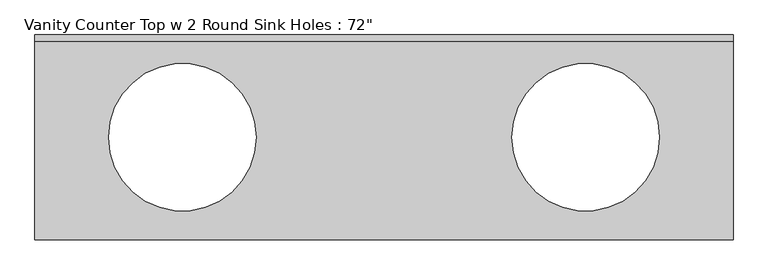
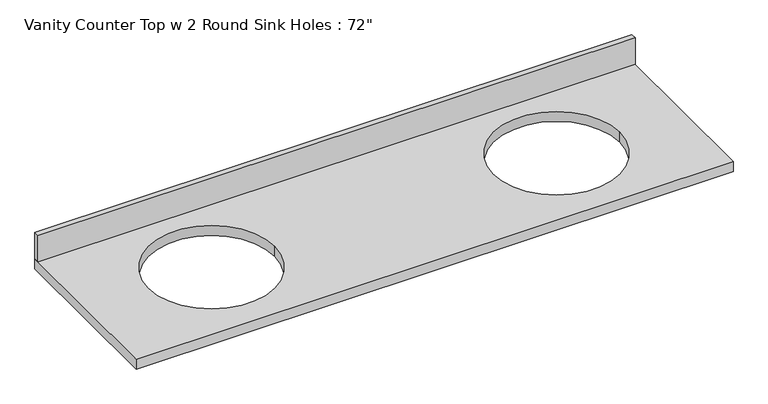
"""IFC4 building model written with IfcOpenShell, lengths in millimetres: furniture geometry."""

import ifcopenshell
import ifcopenshell.guid

model = None  # the IFC model being written
_history = None  # IfcOwnerHistory: only IFC2X3 demands one
_inside = {}  # id of a spatial element -> (the spatial element, [elements in it])
_under = {}  # id of a project, library or spatial element -> (it, [spatial elements below it])
_declared = {}  # id of a project -> (the project, [libraries it declares])
_typed = {}  # id of a type object -> (the type object, [elements of that type])
_made_of = {}  # id of a material, layer set ... -> (it, [elements and type objects made of it])


def new_model(schema):
    """Start an empty IFC model of exactly this schema.

    Asked for "IFC4X3", IfcOpenShell would pick the latest addendum, in which some entities
    have other attributes; the version numbers below select the first issue.
    IFC2X3 requires an IfcOwnerHistory on every rooted entity: one is made here for all.
    """
    global model, _history
    if schema == "IFC4X3":
        model = ifcopenshell.file(schema_version=(4, 3, 0, 0))
    else:
        model = ifcopenshell.file(schema=schema)
    _inside.clear()
    _under.clear()
    _declared.clear()
    _typed.clear()
    _made_of.clear()
    _history = None
    if model.schema == "IFC2X3":
        org = make("IfcOrganization", Name="unknown")
        user = make(
            "IfcPersonAndOrganization",
            ThePerson=make("IfcPerson", FamilyName="unknown"),
            TheOrganization=org,
        )
        app = make(
            "IfcApplication",
            ApplicationDeveloper=org,
            Version="unknown",
            ApplicationFullName="unknown",
            ApplicationIdentifier="unknown",
        )
        _history = make(
            "IfcOwnerHistory",
            OwningUser=user,
            OwningApplication=app,
            ChangeAction="ADDED",
            CreationDate=0,
        )
    return model


def make(cls, **values):
    """One entity of the class cls with the attributes given. An attribute that is None is left unset."""
    return model.create_entity(
        cls, **{name: value for name, value in values.items() if value is not None}
    )


def rooted(cls, **values):
    """An entity with a GlobalId (a new one), such as an element, a storey or a relation."""
    return make(cls, GlobalId=ifcopenshell.guid.new(), OwnerHistory=_history, **values)


def si_unit(unit_type, name, prefix=None):
    """IfcSIUnit, for example si_unit("LENGTHUNIT", "METRE", prefix="MILLI")."""
    return make("IfcSIUnit", UnitType=unit_type, Prefix=prefix, Name=name)


def assignment(units):
    """IfcUnitAssignment: the units of a project."""
    return None if units is None else make("IfcUnitAssignment", Units=units)


def point(xyz):
    """IfcCartesianPoint."""
    return None if xyz is None else make("IfcCartesianPoint", Coordinates=xyz)


def direction(xyz):
    """IfcDirection."""
    return None if xyz is None else make("IfcDirection", DirectionRatios=xyz)


def frame(location, z_axis=None, x_axis=None):
    """IfcAxis2Placement3D, a coordinate frame: its origin and axes. An axis left out is left unset."""
    return make(
        "IfcAxis2Placement3D",
        Location=point(location),
        Axis=direction(z_axis),
        RefDirection=direction(x_axis),
    )


def frame_2d(location, x_axis=None):
    """IfcAxis2Placement2D, a coordinate frame in the plane: its origin and x axis."""
    return make(
        "IfcAxis2Placement2D", Location=point(location), RefDirection=direction(x_axis)
    )


def origin():
    """The frame at (0, 0, 0) with its axes left unset."""
    return frame((0.0, 0.0, 0.0))


def place(relative_to, where):
    """IfcLocalPlacement: puts the frame where relative to a parent placement (None: the world)."""
    return make(
        "IfcLocalPlacement", PlacementRelTo=relative_to, RelativePlacement=where
    )


def context(
    kind, dimensions, precision=None, world=None, true_north=None, identifier=None
):
    """IfcGeometricRepresentationContext, for example the 3D "Model" context."""
    return make(
        "IfcGeometricRepresentationContext",
        ContextIdentifier=identifier,
        ContextType=kind,
        CoordinateSpaceDimension=dimensions,
        Precision=precision,
        WorldCoordinateSystem=world,
        TrueNorth=true_north,
    )


def project(units=None, contexts=None):
    """IfcProject with its units and contexts."""
    return rooted(
        "IfcProject",
        Name="project",
        RepresentationContexts=contexts,
        UnitsInContext=assignment(units),
    )


def spatial(cls, under=None, at=None, **own):
    """A site, building, storey or space (cls), placed at a placement, below another one or the project."""
    s = rooted(cls, ObjectPlacement=at, **own)
    if under is not None:
        _under.setdefault(under.id(), (under, []))[1].append(s)
    return s


def polyline(points):
    """IfcPolyline through the points."""
    return make("IfcPolyline", Points=[point(p) for p in points])


def circle_curve(where, radius):
    """IfcCircle in the frame where."""
    return make("IfcCircle", Position=where, Radius=radius)


def trimmed(basis, trim1, trim2, sense, master):
    """IfcTrimmedCurve: the piece of a basis curve between two trims."""
    return make(
        "IfcTrimmedCurve",
        BasisCurve=basis,
        Trim1=trim1,
        Trim2=trim2,
        SenseAgreement=sense,
        MasterRepresentation=master,
    )


def segment(curve, same_sense, transition):
    """IfcCompositeCurveSegment."""
    return make(
        "IfcCompositeCurveSegment",
        Transition=transition,
        SameSense=same_sense,
        ParentCurve=curve,
    )


def composite_curve(segments, self_intersect=None):
    """IfcCompositeCurve: segments joined end to end."""
    return make("IfcCompositeCurve", Segments=segments, SelfIntersect=self_intersect)


def outline(outer, holes=None, kind="AREA"):
    """IfcArbitraryClosedProfileDef: a profile drawn as a closed curve; with holes, ...WithVoids."""
    if holes is None:
        return make("IfcArbitraryClosedProfileDef", ProfileType=kind, OuterCurve=outer)
    return make(
        "IfcArbitraryProfileDefWithVoids",
        ProfileType=kind,
        OuterCurve=outer,
        InnerCurves=holes,
    )


def extrude(swept, where, along, depth):
    """IfcExtrudedAreaSolid: the profile swept, set in the frame where, extruded along a direction by depth."""
    return make(
        "IfcExtrudedAreaSolid",
        SweptArea=swept,
        Position=where,
        ExtrudedDirection=direction(along),
        Depth=depth,
    )


def shape(context_of_items, identifier, shape_type, items):
    """IfcShapeRepresentation: the items that make up one representation, for example the "Body"."""
    return make(
        "IfcShapeRepresentation",
        ContextOfItems=context_of_items,
        RepresentationIdentifier=identifier,
        RepresentationType=shape_type,
        Items=items,
    )


def source(mapping_origin, context_of_items, identifier, shape_type, items):
    """IfcRepresentationMap: a shape defined once, which mapped items show again and again."""
    return make(
        "IfcRepresentationMap",
        MappingOrigin=mapping_origin,
        MappedRepresentation=shape(context_of_items, identifier, shape_type, items),
    )


def transform(
    local_origin,
    x_axis=None,
    y_axis=None,
    z_axis=None,
    scale=None,
    scale2=None,
    scale3=None,
    uniform=True,
):
    """IfcCartesianTransformationOperator3D, or its non-uniform kind. x_axis, y_axis, z_axis: its Axis1, 2, 3."""
    if uniform:
        return make(
            "IfcCartesianTransformationOperator3D",
            Axis1=direction(x_axis),
            Axis2=direction(y_axis),
            LocalOrigin=point(local_origin),
            Scale=scale,
            Axis3=direction(z_axis),
        )
    return make(
        "IfcCartesianTransformationOperator3DnonUniform",
        Axis1=direction(x_axis),
        Axis2=direction(y_axis),
        LocalOrigin=point(local_origin),
        Scale=scale,
        Axis3=direction(z_axis),
        Scale2=scale2,
        Scale3=scale3,
    )


def mapped(mapping_source, mapping_target):
    """IfcMappedItem: shows the shape of a source again, moved by a transform."""
    return make(
        "IfcMappedItem", MappingSource=mapping_source, MappingTarget=mapping_target
    )


def made_of(thing, what):
    """Note that an element or type object is made of a material, layer set ...; save() writes the relation."""
    if what is not None:
        _made_of.setdefault(what.id(), (what, []))[1].append(thing)
    return thing


def element(
    cls,
    number,
    at=None,
    inside=None,
    cuts=None,
    type_object=None,
    material=None,
    context=None,
    identifier="Body",
    shape_type=None,
    held_by="IfcProductDefinitionShape",
    body=None,
    shapes=None,
    **own,
):
    """One element of the class cls, such as IfcWall. Its Tag is "e" and its number.

    at: its placement. inside: the storey or other place that contains it. cuts: it is an
    opening in that element (IfcRelVoidsElement). A single representation is given by context,
    identifier, shape_type and body (its items); several are given by shapes. held_by: the class
    of the entity that holds the representations. save() writes the other relations.
    """
    e = rooted(cls, Tag="e%d" % number, ObjectPlacement=at, **own)
    if body is not None:
        shapes = [shape(context, identifier, shape_type, body)]
    if shapes is not None:
        e.Representation = make(held_by, Representations=shapes)
    if inside is not None:
        _inside.setdefault(inside.id(), (inside, []))[1].append(e)
    if cuts is not None:
        rooted(
            "IfcRelVoidsElement", RelatingBuildingElement=cuts, RelatedOpeningElement=e
        )
    if type_object is not None:
        _typed.setdefault(type_object.id(), (type_object, []))[1].append(e)
    return made_of(e, material)


def aggregate(whole, parts):
    """IfcRelAggregates: a whole, such as a stair, and the parts it consists of."""
    return rooted("IfcRelAggregates", RelatingObject=whole, RelatedObjects=parts)


def save(model, path):
    """Write the relations noted so far, then the file.

    IfcRelAggregates (storeys below a building ...), IfcRelContainedInSpatialStructure (elements
    in a storey), IfcRelDefinesByType, IfcRelAssociatesMaterial and IfcRelDeclares: one each for
    every whole, place, type object, material and project.
    """
    for whole, parts in _under.values():
        aggregate(whole, parts)
    for where, things in _inside.values():
        rooted(
            "IfcRelContainedInSpatialStructure",
            RelatedElements=things,
            RelatingStructure=where,
        )
    for kind, things in _typed.values():
        rooted("IfcRelDefinesByType", RelatedObjects=things, RelatingType=kind)
    for what, things in _made_of.values():
        rooted("IfcRelAssociatesMaterial", RelatedObjects=things, RelatingMaterial=what)
    for by, libraries in _declared.values():
        rooted("IfcRelDeclares", RelatingContext=by, RelatedDefinitions=libraries)
    model.write(path)


def furniture_635471ae(model_context):
    return source(origin(), model_context, "Body", "SweptSolid", [
        extrude(outline(polyline([(-1327.4622951, 0.0), (837.8877049, 0.0), (837.8877049, -19.05), (-1327.4622951, -19.05), (-1327.4622951, 0.0)])), frame((0.0, 0.0, 787.4), z_axis=(0.0, 0.0, 1.0), x_axis=(1.0, 0.0, 0.0)), (0.0, 0.0, 1.0), 101.6),
        extrude(outline(polyline([(837.8877049, 0.0), (837.8877049, -635.0), (-1327.4622951, -635.0), (-1327.4622951, 0.0), (837.8877049, 0.0)]), holes=[composite_curve([segment(trimmed(circle_curve(frame_2d((-870.2622951, -317.5)), 228.6), [point((-1098.8622951, -317.5))], [point((-641.6622951, -317.5))], True, "CARTESIAN"), True, "CONTINUOUS"), segment(trimmed(circle_curve(frame_2d((-870.2622951, -317.5)), 228.6), [point((-641.6622951, -317.5))], [point((-1098.8622951, -317.5))], True, "CARTESIAN"), True, "CONTINUOUS")], self_intersect=False), composite_curve([segment(trimmed(circle_curve(frame_2d((380.6877049, -317.5)), 228.6), [point((152.0877049, -317.5))], [point((609.2877049, -317.5))], True, "CARTESIAN"), True, "CONTINUOUS"), segment(trimmed(circle_curve(frame_2d((380.6877049, -317.5)), 228.6), [point((609.2877049, -317.5))], [point((152.0877049, -317.5))], True, "CARTESIAN"), True, "CONTINUOUS")], self_intersect=False)]), frame((0.0, 0.0, 749.3), z_axis=(0.0, 0.0, 1.0), x_axis=(1.0, 0.0, 0.0)), (0.0, 0.0, 1.0), 38.1),
    ])


if __name__ == "__main__":
    model = new_model("IFC4")
    model_context = context("Model", 3, world=origin())
    ifc_project = project(units=[si_unit("LENGTHUNIT", "METRE", prefix="MILLI")], contexts=[model_context])
    site = spatial("IfcSite", under=ifc_project)
    building = spatial("IfcBuilding", under=site)
    placement = place(None, origin())
    furniture_shape = furniture_635471ae(model_context)
    element("IfcFurniture", 1, ObjectType="Vanity Counter Top w 2 Round Sink Holes : 72\"", at=placement, inside=building, context=model_context, shape_type="MappedRepresentation", body=[
        mapped(furniture_shape, transform((0.0, 0.0, 0.0), x_axis=(1.0, 0.0, 0.0), y_axis=(0.0, 1.0, 0.0), z_axis=(0.0, 0.0, 1.0))),
    ])
    save(model, "model.ifc")

# Revit data of these elements
# Type "Vanity Counter Top w 2 Round Sink Holes : 72\""
#   Assembly Code = "C1030400"
#   Sink Location Right = 1' - 6"
#   Counter Thickness = 0' - 1 1/2"
#   Depth = 2' - 1"
#   Height = 2' - 7"
#   Length [instance default] = 6' - 0"
#   Sink Location Left [instance default] = 1' - 6"
#   Sink Location To Wall [instance default] = 0' - 4"
#   Sink Opening Width [instance default] = 1' - 5"
#   Counter Top = Counter Top
# Element 1 (IfcFurniture, "Vanity Counter Top w 2 Round Sink Holes : 72\"")
#   Length = 7' - 1 1/4"
#   Materials on its faces: "Counter Top"
# Materials
#   "Counter Top": class "Wood", colour RGB 226 177 128, transparency 0
